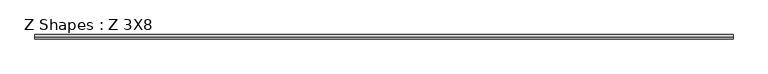
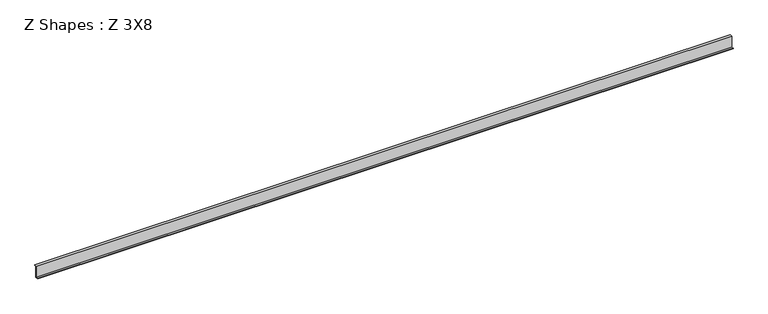
"""IFC4 building model written with IfcOpenShell, lengths in millimetres: beam geometry, Z Shapes : Z 3X8."""

from ifc_helpers import new_model, si_unit, frame, origin, place, context, project, spatial, polyline, outline, extrude, source, transform, mapped, element, save


def z_shapes_z_3x8_9800e643(model_context):
    return source(origin(), model_context, "Body", "SweptSolid", [
        extrude(outline(polyline([(57.2805719, 92.452825), (27.1991352, 92.452825), (27.1991352, -98.809175), (-18.9194281, -98.809175), (-18.9194281, -92.459175), (19.1805719, -92.459175), (19.1805719, 102.104825), (57.2805719, 102.104825), (57.2805719, 92.452825)])), frame((-5835.65, 0.0, 0.0), z_axis=(1.0, 0.0, 0.0), x_axis=(0.0, 1.0, 0.0)), (0.0, 0.0, 1.0), 11671.3),
    ])


if __name__ == "__main__":
    model = new_model("IFC4")
    model_context = context("Model", 3, world=origin())
    ifc_project = project(units=[si_unit("LENGTHUNIT", "METRE", prefix="MILLI")], contexts=[model_context])
    site = spatial("IfcSite", under=ifc_project)
    building = spatial("IfcBuilding", under=site)
    placement = place(None, origin())
    z_shapes_z_3x8_shape = z_shapes_z_3x8_9800e643(model_context)
    element("IfcBeam", 1, ObjectType="Z Shapes : Z 3X8", at=placement, inside=building, context=model_context, shape_type="MappedRepresentation", body=[
        mapped(z_shapes_z_3x8_shape, transform((0.0, 0.0, 0.0), x_axis=(1.0, 0.0, 0.0), y_axis=(0.0, 1.0, 0.0), z_axis=(0.0, 0.0, 1.0))),
    ])
    save(model, "model.ifc")

# Revit data of these elements
# Type "Z Shapes : Z 3X8"
#   Section Name Key = "W12x26"
#   Assembly Code = "B10"
#   Width = 76.2 mm
#   Web Thickness = 5.842 mm
#   Web Fillet = 7.62 mm
#   Warping Constant = 163001.3 cm⁶
#   Torsional Moment of Inertia = 12.4869 cm⁴
#   Section Area = 7.65 in²
#   Plastic Modulus weak axis = 0.00472801 (stored number, unit not read)
#   Plastic Modulus strong axis = 0.0215278 (stored number, unit not read)
#   Perimeter = 15.0571 m²/m
#   Nominal Weight = 379.441 N/m
#   Moment of Inertia weak axis = 720.08 cm⁴
#   Moment of Inertia strong axis = 8491.12 cm⁴
#   Height = 184.912 mm
#   Flange Thickness = 9.652 mm
#   Elastic Modulus weak axis = 0.00309028 (stored number, unit not read)
#   Elastic Modulus strong axis = 0.0193287 (stored number, unit not read)
#   Centroid Vertical = 92.456 mm
#   Centroid Horizontal = 38.1 mm
#   Length [instance default] = 5' - 0"
#   Structural Material [instance default] = Steel ASTM A992
#   Principal Axes Angle = 0
# Element 1 (IfcBeam, "Z Shapes : Z 3X8")
#   Structural Material = accent 2
#   Materials on its faces: "accent 2"
# Materials
#   "Steel ASTM A992": class "Metal", colour RGB 189 187 185, transparency 0, Description = "Structural steel 50ksi", Cost = 0
#   "accent 2": class "Wood", colour RGB 80 80 80, transparency 0, Description = "Wood framing, thermal airspace", Cost = 0
